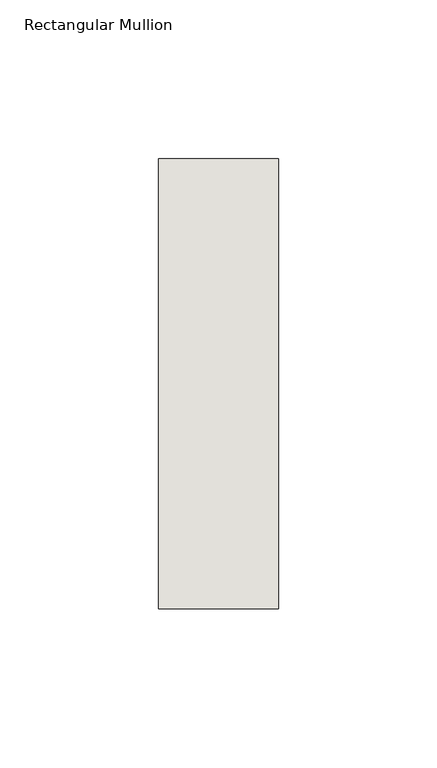
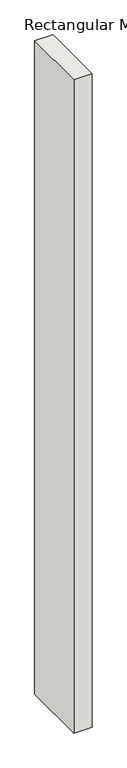
"""IFC4 building model written with IfcOpenShell, lengths in millimetres: wall geometry, Rectangular Mullion : NLRS_21_CWM_hsb-regel 38x142_gen_rsf."""

from ifc_helpers import new_model, si_unit, frame, origin, place, context, project, spatial, polyline, outline, extrude, source, transform, mapped, element, save


def rectangular_mullion_de1563bf(model_context):
    return source(origin(), model_context, "Body", "SweptSolid", [
        extrude(outline(polyline([(0.0, -71.0), (-38.0, -71.0), (-38.0, 71.0), (0.0, 71.0), (0.0, -71.0)])), frame((0.0, 0.0, -1440.0), z_axis=(0.0, 0.0, 1.0), x_axis=(1.0, 0.0, 0.0)), (0.0, 0.0, 1.0), 1440.0),
    ])


if __name__ == "__main__":
    model = new_model("IFC4")
    model_context = context("Model", 3, world=origin())
    ifc_project = project(units=[si_unit("LENGTHUNIT", "METRE", prefix="MILLI")], contexts=[model_context])
    site = spatial("IfcSite", under=ifc_project)
    building = spatial("IfcBuilding", under=site)
    placement = place(None, origin())
    rectangular_mullion_shape = rectangular_mullion_de1563bf(model_context)
    element("IfcWall", 1, ObjectType="Rectangular Mullion : NLRS_21_CWM_hsb-regel 38x142_gen_rsf", at=placement, inside=building, context=model_context, shape_type="MappedRepresentation", body=[
        mapped(rectangular_mullion_shape, transform((0.0, 0.0, 0.0), x_axis=(1.0, 0.0, 0.0), y_axis=(0.0, 1.0, 0.0), z_axis=(0.0, 0.0, 1.0))),
    ])
    save(model, "model.ifc")

# Revit data of these elements
# Type "Rectangular Mullion : NLRS_21_CWM_hsb-regel 38x142_gen_rsf"
#   Type IfcGUID = "07M7mRoiH1CR8m_RSKIwpF"
#   Assembly Code = "21.10"
#   IfcExportAs = "IfcWall"
#   built-in parameter 1007322 = 0.465879 (stored number, unit not read)
#   built-in parameter 1007321 = 0.062336 (stored number, unit not read)
#   built-in parameter 1007320 = 0.062336 (stored number, unit not read)
# Element 1 (IfcWall, "Rectangular Mullion : NLRS_21_CWM_hsb-regel 38x142_gen_rsf")
#   Materials on its faces: "NLRS_i2_hout naaldhout vuren_gen_rsf"
# Materials
#   "NLRS_i2_hout naaldhout vuren_gen_rsf": class "I - Hout", colour RGB 234 199 147, transparency 0, Keynote = "i2", Manufacturer = "Revit Standards Foundation", URL = "www.revitstandards.org", Description = "hout vuren", Cost = 0
